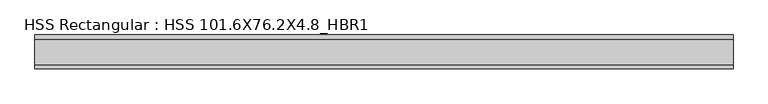
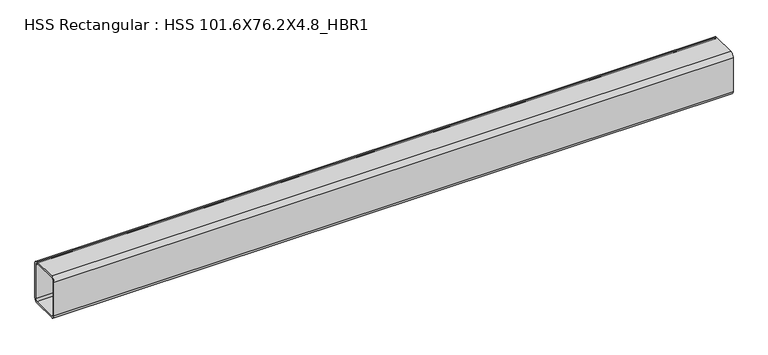
"""IFC4 building model written with IfcOpenShell, lengths in millimetres: beam geometry, HSS Rectangular : HSS 101.6X76.2X4.8_HBR1."""

import ifcopenshell
import ifcopenshell.guid

model = None  # the IFC model being written
_history = None  # IfcOwnerHistory: only IFC2X3 demands one
_inside = {}  # id of a spatial element -> (the spatial element, [elements in it])
_under = {}  # id of a project, library or spatial element -> (it, [spatial elements below it])
_declared = {}  # id of a project -> (the project, [libraries it declares])
_typed = {}  # id of a type object -> (the type object, [elements of that type])
_made_of = {}  # id of a material, layer set ... -> (it, [elements and type objects made of it])


def new_model(schema):
    """Start an empty IFC model of exactly this schema.

    Asked for "IFC4X3", IfcOpenShell would pick the latest addendum, in which some entities
    have other attributes; the version numbers below select the first issue.
    IFC2X3 requires an IfcOwnerHistory on every rooted entity: one is made here for all.
    """
    global model, _history
    if schema == "IFC4X3":
        model = ifcopenshell.file(schema_version=(4, 3, 0, 0))
    else:
        model = ifcopenshell.file(schema=schema)
    _inside.clear()
    _under.clear()
    _declared.clear()
    _typed.clear()
    _made_of.clear()
    _history = None
    if model.schema == "IFC2X3":
        org = make("IfcOrganization", Name="unknown")
        user = make(
            "IfcPersonAndOrganization",
            ThePerson=make("IfcPerson", FamilyName="unknown"),
            TheOrganization=org,
        )
        app = make(
            "IfcApplication",
            ApplicationDeveloper=org,
            Version="unknown",
            ApplicationFullName="unknown",
            ApplicationIdentifier="unknown",
        )
        _history = make(
            "IfcOwnerHistory",
            OwningUser=user,
            OwningApplication=app,
            ChangeAction="ADDED",
            CreationDate=0,
        )
    return model


def make(cls, **values):
    """One entity of the class cls with the attributes given. An attribute that is None is left unset."""
    return model.create_entity(
        cls, **{name: value for name, value in values.items() if value is not None}
    )


def rooted(cls, **values):
    """An entity with a GlobalId (a new one), such as an element, a storey or a relation."""
    return make(cls, GlobalId=ifcopenshell.guid.new(), OwnerHistory=_history, **values)


def si_unit(unit_type, name, prefix=None):
    """IfcSIUnit, for example si_unit("LENGTHUNIT", "METRE", prefix="MILLI")."""
    return make("IfcSIUnit", UnitType=unit_type, Prefix=prefix, Name=name)


def assignment(units):
    """IfcUnitAssignment: the units of a project."""
    return None if units is None else make("IfcUnitAssignment", Units=units)


def point(xyz):
    """IfcCartesianPoint."""
    return None if xyz is None else make("IfcCartesianPoint", Coordinates=xyz)


def direction(xyz):
    """IfcDirection."""
    return None if xyz is None else make("IfcDirection", DirectionRatios=xyz)


def frame(location, z_axis=None, x_axis=None):
    """IfcAxis2Placement3D, a coordinate frame: its origin and axes. An axis left out is left unset."""
    return make(
        "IfcAxis2Placement3D",
        Location=point(location),
        Axis=direction(z_axis),
        RefDirection=direction(x_axis),
    )


def frame_2d(location, x_axis=None):
    """IfcAxis2Placement2D, a coordinate frame in the plane: its origin and x axis."""
    return make(
        "IfcAxis2Placement2D", Location=point(location), RefDirection=direction(x_axis)
    )


def origin():
    """The frame at (0, 0, 0) with its axes left unset."""
    return frame((0.0, 0.0, 0.0))


def place(relative_to, where):
    """IfcLocalPlacement: puts the frame where relative to a parent placement (None: the world)."""
    return make(
        "IfcLocalPlacement", PlacementRelTo=relative_to, RelativePlacement=where
    )


def context(
    kind, dimensions, precision=None, world=None, true_north=None, identifier=None
):
    """IfcGeometricRepresentationContext, for example the 3D "Model" context."""
    return make(
        "IfcGeometricRepresentationContext",
        ContextIdentifier=identifier,
        ContextType=kind,
        CoordinateSpaceDimension=dimensions,
        Precision=precision,
        WorldCoordinateSystem=world,
        TrueNorth=true_north,
    )


def project(units=None, contexts=None):
    """IfcProject with its units and contexts."""
    return rooted(
        "IfcProject",
        Name="project",
        RepresentationContexts=contexts,
        UnitsInContext=assignment(units),
    )


def spatial(cls, under=None, at=None, **own):
    """A site, building, storey or space (cls), placed at a placement, below another one or the project."""
    s = rooted(cls, ObjectPlacement=at, **own)
    if under is not None:
        _under.setdefault(under.id(), (under, []))[1].append(s)
    return s


def polyline(points):
    """IfcPolyline through the points."""
    return make("IfcPolyline", Points=[point(p) for p in points])


def circle_curve(where, radius):
    """IfcCircle in the frame where."""
    return make("IfcCircle", Position=where, Radius=radius)


def trimmed(basis, trim1, trim2, sense, master):
    """IfcTrimmedCurve: the piece of a basis curve between two trims."""
    return make(
        "IfcTrimmedCurve",
        BasisCurve=basis,
        Trim1=trim1,
        Trim2=trim2,
        SenseAgreement=sense,
        MasterRepresentation=master,
    )


def segment(curve, same_sense, transition):
    """IfcCompositeCurveSegment."""
    return make(
        "IfcCompositeCurveSegment",
        Transition=transition,
        SameSense=same_sense,
        ParentCurve=curve,
    )


def composite_curve(segments, self_intersect=None):
    """IfcCompositeCurve: segments joined end to end."""
    return make("IfcCompositeCurve", Segments=segments, SelfIntersect=self_intersect)


def outline(outer, holes=None, kind="AREA"):
    """IfcArbitraryClosedProfileDef: a profile drawn as a closed curve; with holes, ...WithVoids."""
    if holes is None:
        return make("IfcArbitraryClosedProfileDef", ProfileType=kind, OuterCurve=outer)
    return make(
        "IfcArbitraryProfileDefWithVoids",
        ProfileType=kind,
        OuterCurve=outer,
        InnerCurves=holes,
    )


def extrude(swept, where, along, depth):
    """IfcExtrudedAreaSolid: the profile swept, set in the frame where, extruded along a direction by depth."""
    return make(
        "IfcExtrudedAreaSolid",
        SweptArea=swept,
        Position=where,
        ExtrudedDirection=direction(along),
        Depth=depth,
    )


def shape(context_of_items, identifier, shape_type, items):
    """IfcShapeRepresentation: the items that make up one representation, for example the "Body"."""
    return make(
        "IfcShapeRepresentation",
        ContextOfItems=context_of_items,
        RepresentationIdentifier=identifier,
        RepresentationType=shape_type,
        Items=items,
    )


def source(mapping_origin, context_of_items, identifier, shape_type, items):
    """IfcRepresentationMap: a shape defined once, which mapped items show again and again."""
    return make(
        "IfcRepresentationMap",
        MappingOrigin=mapping_origin,
        MappedRepresentation=shape(context_of_items, identifier, shape_type, items),
    )


def transform(
    local_origin,
    x_axis=None,
    y_axis=None,
    z_axis=None,
    scale=None,
    scale2=None,
    scale3=None,
    uniform=True,
):
    """IfcCartesianTransformationOperator3D, or its non-uniform kind. x_axis, y_axis, z_axis: its Axis1, 2, 3."""
    if uniform:
        return make(
            "IfcCartesianTransformationOperator3D",
            Axis1=direction(x_axis),
            Axis2=direction(y_axis),
            LocalOrigin=point(local_origin),
            Scale=scale,
            Axis3=direction(z_axis),
        )
    return make(
        "IfcCartesianTransformationOperator3DnonUniform",
        Axis1=direction(x_axis),
        Axis2=direction(y_axis),
        LocalOrigin=point(local_origin),
        Scale=scale,
        Axis3=direction(z_axis),
        Scale2=scale2,
        Scale3=scale3,
    )


def mapped(mapping_source, mapping_target):
    """IfcMappedItem: shows the shape of a source again, moved by a transform."""
    return make(
        "IfcMappedItem", MappingSource=mapping_source, MappingTarget=mapping_target
    )


def made_of(thing, what):
    """Note that an element or type object is made of a material, layer set ...; save() writes the relation."""
    if what is not None:
        _made_of.setdefault(what.id(), (what, []))[1].append(thing)
    return thing


def element(
    cls,
    number,
    at=None,
    inside=None,
    cuts=None,
    type_object=None,
    material=None,
    context=None,
    identifier="Body",
    shape_type=None,
    held_by="IfcProductDefinitionShape",
    body=None,
    shapes=None,
    **own,
):
    """One element of the class cls, such as IfcWall. Its Tag is "e" and its number.

    at: its placement. inside: the storey or other place that contains it. cuts: it is an
    opening in that element (IfcRelVoidsElement). A single representation is given by context,
    identifier, shape_type and body (its items); several are given by shapes. held_by: the class
    of the entity that holds the representations. save() writes the other relations.
    """
    e = rooted(cls, Tag="e%d" % number, ObjectPlacement=at, **own)
    if body is not None:
        shapes = [shape(context, identifier, shape_type, body)]
    if shapes is not None:
        e.Representation = make(held_by, Representations=shapes)
    if inside is not None:
        _inside.setdefault(inside.id(), (inside, []))[1].append(e)
    if cuts is not None:
        rooted(
            "IfcRelVoidsElement", RelatingBuildingElement=cuts, RelatedOpeningElement=e
        )
    if type_object is not None:
        _typed.setdefault(type_object.id(), (type_object, []))[1].append(e)
    return made_of(e, material)


def aggregate(whole, parts):
    """IfcRelAggregates: a whole, such as a stair, and the parts it consists of."""
    return rooted("IfcRelAggregates", RelatingObject=whole, RelatedObjects=parts)


def save(model, path):
    """Write the relations noted so far, then the file.

    IfcRelAggregates (storeys below a building ...), IfcRelContainedInSpatialStructure (elements
    in a storey), IfcRelDefinesByType, IfcRelAssociatesMaterial and IfcRelDeclares: one each for
    every whole, place, type object, material and project.
    """
    for whole, parts in _under.values():
        aggregate(whole, parts)
    for where, things in _inside.values():
        rooted(
            "IfcRelContainedInSpatialStructure",
            RelatedElements=things,
            RelatingStructure=where,
        )
    for kind, things in _typed.values():
        rooted("IfcRelDefinesByType", RelatedObjects=things, RelatingType=kind)
    for what, things in _made_of.values():
        rooted("IfcRelAssociatesMaterial", RelatedObjects=things, RelatingMaterial=what)
    for by, libraries in _declared.values():
        rooted("IfcRelDeclares", RelatingContext=by, RelatedDefinitions=libraries)
    model.write(path)


def hss_rectangular_hss_101_6x76_2x4_8_hbr1_19457b14(model_context):
    return source(origin(), model_context, "Body", "SweptSolid", [
        extrude(outline(composite_curve([segment(polyline([(38.1, 41.275), (38.1, -41.275)]), True, "CONTINUOUS"), segment(trimmed(circle_curve(frame_2d((28.575, -41.275)), 9.525), [point((38.1, -41.275))], [point((28.575, -50.8))], False, "CARTESIAN"), True, "CONTINUOUS"), segment(polyline([(28.575, -50.8), (-28.575, -50.8)]), True, "CONTINUOUS"), segment(trimmed(circle_curve(frame_2d((-28.575, -41.275)), 9.525), [point((-28.575, -50.8))], [point((-38.1, -41.275))], False, "CARTESIAN"), True, "CONTINUOUS"), segment(polyline([(-38.1, -41.275), (-38.1, 41.275)]), True, "CONTINUOUS"), segment(trimmed(circle_curve(frame_2d((-28.575, 41.275)), 9.525), [point((-38.1, 41.275))], [point((-28.575, 50.8))], False, "CARTESIAN"), True, "CONTINUOUS"), segment(polyline([(-28.575, 50.8), (28.575, 50.8)]), True, "CONTINUOUS"), segment(trimmed(circle_curve(frame_2d((28.575, 41.275)), 9.525), [point((28.575, 50.8))], [point((38.1, 41.275))], False, "CARTESIAN"), True, "CONTINUOUS")], self_intersect=False), holes=[composite_curve([segment(trimmed(circle_curve(frame_2d((-28.575, 41.275)), 4.7625), [point((-28.575, 46.0375))], [point((-33.3375, 41.275))], True, "CARTESIAN"), True, "CONTINUOUS"), segment(polyline([(-33.3375, 41.275), (-33.3375, -41.275)]), True, "CONTINUOUS"), segment(trimmed(circle_curve(frame_2d((-28.575, -41.275)), 4.7625), [point((-33.3375, -41.275))], [point((-28.575, -46.0375))], True, "CARTESIAN"), True, "CONTINUOUS"), segment(polyline([(-28.575, -46.0375), (28.575, -46.0375)]), True, "CONTINUOUS"), segment(trimmed(circle_curve(frame_2d((28.575, -41.275)), 4.7625), [point((28.575, -46.0375))], [point((33.3375, -41.275))], True, "CARTESIAN"), True, "CONTINUOUS"), segment(polyline([(33.3375, -41.275), (33.3375, 41.275)]), True, "CONTINUOUS"), segment(trimmed(circle_curve(frame_2d((28.575, 41.275)), 4.7625), [point((33.3375, 41.275))], [point((28.575, 46.0375))], True, "CARTESIAN"), True, "CONTINUOUS"), segment(polyline([(28.575, 46.0375), (-28.575, 46.0375)]), True, "CONTINUOUS")], self_intersect=False)]), frame((-719.0409044, 0.0, 0.0), z_axis=(1.0, 0.0, 0.0), x_axis=(0.0, 1.0, 0.0)), (0.0, 0.0, 1.0), 1569.0409044),
    ])


if __name__ == "__main__":
    model = new_model("IFC4")
    model_context = context("Model", 3, world=origin())
    ifc_project = project(units=[si_unit("LENGTHUNIT", "METRE", prefix="MILLI")], contexts=[model_context])
    site = spatial("IfcSite", under=ifc_project)
    building = spatial("IfcBuilding", under=site)
    placement = place(None, origin())
    hss_rectangular_hss_101_6x76_2x4_8_hbr1_shape = hss_rectangular_hss_101_6x76_2x4_8_hbr1_19457b14(model_context)
    element("IfcBeam", 1, ObjectType="HSS Rectangular : HSS 101.6X76.2X4.8_HBR1", at=placement, inside=building, context=model_context, shape_type="MappedRepresentation", body=[
        mapped(hss_rectangular_hss_101_6x76_2x4_8_hbr1_shape, transform((0.0, 0.0, 0.0), x_axis=(1.0, 0.0, 0.0), y_axis=(0.0, 1.0, 0.0), z_axis=(0.0, 0.0, 1.0))),
    ])
    save(model, "model.ifc")

# Revit data of these elements
# Type "HSS Rectangular : HSS 101.6X76.2X4.8_HBR1"
#   Section Name Key = "HSS 4X3X3/16"
#   Assembly Code = "B10"
#   Width = 7.62 cm
#   Wall Nominal Thickness = 0.4763 cm
#   Wall Design Thickness = 0.442 cm
#   Torsional Moment of Inertia = 260.561 cm⁴
#   Torsional Modulus = 61.2876 cm³
#   Section Area = 14.4516 cm²
#   Plastic Modulus weak axis = 40.3122 cm³
#   Plastic Modulus strong axis = 49.1612 cm³
#   Perimeter = 0.881482 m²/m
#   Outer Fillet = 0.9525 cm
#   Nominal Weight = 12.1285 kgf/m
#   Moment of Inertia weak axis = 131.529 cm⁴
#   Moment of Inertia strong axis = 205.202 cm⁴
#   Inner Fillet = 0.4763 cm
#   Height = 10.16 cm
#   Elastic Modulus weak axis = 34.4128 cm³
#   Elastic Modulus strong axis = 40.476 cm³
#   Centroid Vertical = 5.08 cm
#   Centroid Horizontal = 3.81 cm
#   Length [instance default] = 1524 mm
#   Structural Material [instance default] = Steel ASTM A500, Grade B, Rectangular and Square
#   Principal Axes Angle = 0
# Element 1 (IfcBeam, "HSS Rectangular : HSS 101.6X76.2X4.8_HBR1")
#   Structural Material = Steel ASTM A992
#   Materials on its faces: "Steel ASTM A992"
# Materials
#   "Steel ASTM A500, Grade B, Rectangular and Square": class "Metal", colour RGB 199 199 199, transparency 0, Description = "Carbon steel", Cost = 0
#   "Steel ASTM A992": class "Metal", colour RGB 199 199 199, transparency 0, Description = "Structural steel 50ksi", Cost = 0
